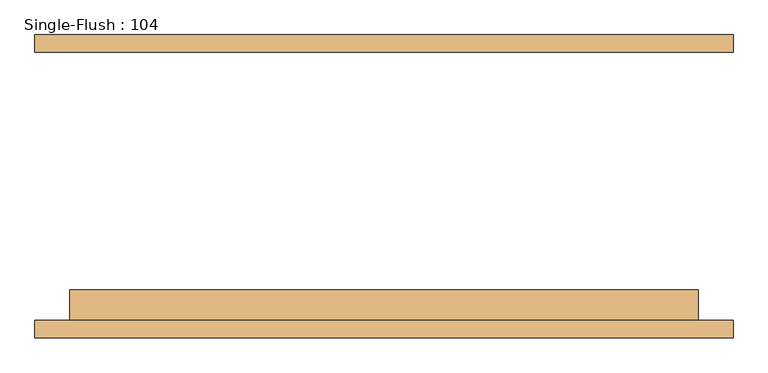
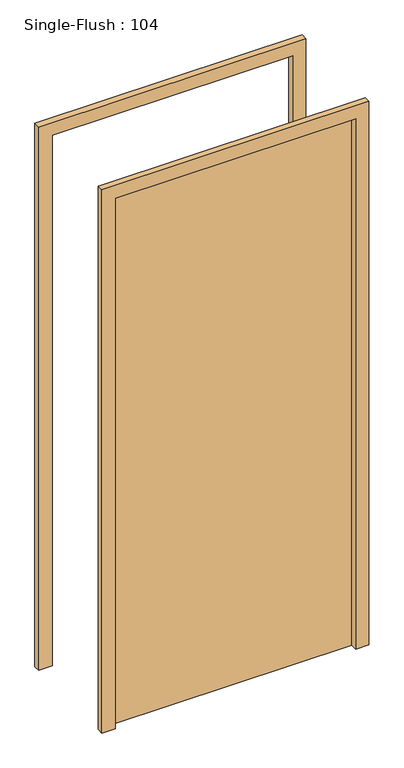
"""IFC4 building model written with IfcOpenShell, lengths in millimetres: door geometry, Single-Flush : 104."""

from ifc_helpers import new_model, si_unit, frame, origin, origin_with_axes, place, context, project, spatial, polyline, outline, extrude, source, transform, mapped, element, save


def single_flush_104_d05c7ce0(model_context):
    return source(origin(), model_context, "Body", "SweptSolid", [
        extrude(outline(polyline([(2184.4, -508.0), (0.0, -508.0), (0.0, -457.2), (2133.6, -457.2), (2133.6, 457.2), (0.0, 457.2), (0.0, 508.0), (2184.4, 508.0), (2184.4, -508.0)])), frame((0.0, -220.6625, 0.0), z_axis=(0.0, 1.0, 0.0), x_axis=(0.0, 0.0, 1.0)), (0.0, 0.0, 1.0), 25.4),
        extrude(outline(polyline([(2184.4, 508.0), (2184.4, -508.0), (0.0, -508.0), (0.0, -457.2), (2133.6, -457.2), (2133.6, 457.2), (0.0, 457.2), (0.0, 508.0), (2184.4, 508.0)])), frame((0.0, 195.2625, 0.0), z_axis=(0.0, 1.0, 0.0), x_axis=(0.0, 0.0, 1.0)), (0.0, 0.0, 1.0), 25.4),
        extrude(outline(polyline([(457.2, -150.8125), (457.2, -195.2625), (-457.2, -195.2625), (-457.2, -150.8125), (457.2, -150.8125)])), origin_with_axes(), (0.0, 0.0, 1.0), 2133.6),
    ])


if __name__ == "__main__":
    model = new_model("IFC4")
    model_context = context("Model", 3, world=origin())
    ifc_project = project(units=[si_unit("LENGTHUNIT", "METRE", prefix="MILLI")], contexts=[model_context])
    site = spatial("IfcSite", under=ifc_project)
    building = spatial("IfcBuilding", under=site)
    placement = place(None, origin())
    single_flush_104_shape = single_flush_104_d05c7ce0(model_context)
    element("IfcDoor", 1, ObjectType="Single-Flush : 104", at=placement, inside=building, context=model_context, shape_type="MappedRepresentation", body=[
        mapped(single_flush_104_shape, transform((0.0, 0.0, 0.0), x_axis=(1.0, 0.0, 0.0), y_axis=(0.0, 1.0, 0.0), z_axis=(0.0, 0.0, 1.0))),
    ])
    save(model, "model.ifc")

# Revit data of these elements
# Type "Single-Flush : 104"
#   Type Mark = "104"
#   Construction Type Id = "MDOOR"
#   Assembly Code = "C1020"
#   Analytic Construction = "Metal"
#   Thickness = 0' - 1 3/4"
#   Heat Transfer Coefficient (U) = 3.7021 W/(m²·K)
#   Height = 7' - 0"
#   Trim Projection Ext = 0' - 1"
#   Trim Projection Int = 0' - 1"
#   Trim Width = 0' - 2"
#   Width = 3' - 0"
#   Door Material = Door - Panel
#   Frame Material = 05 - Metal - Aluminum
#   Visual Light Transmittance = 0
#   Solar Heat Gain Coefficient = 0
#   Function = (empty or 0)
#   Wall Closure = (empty or 0)
# Element 1 (IfcDoor, "Single-Flush : 104")
#   Materials on its faces: "05 - Metal - Aluminum", "Door - Panel"
# Materials
#   "Door - Panel": class "Wood", colour RGB 210 159 95, transparency 0
#   "05 - Metal - Aluminum": class "Unassigned", colour RGB 247 247 247, transparency 0, Description = "Aluminum"
